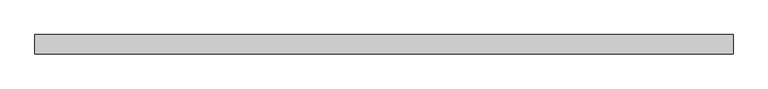
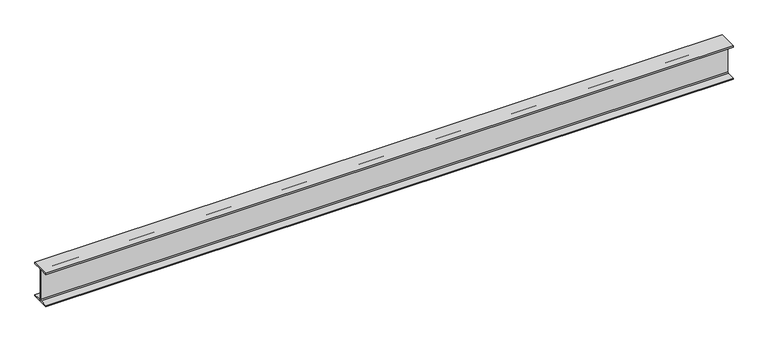
"""IFC4 building model written with IfcOpenShell, lengths in millimetres: beam geometry, Old_Steel Beam_H-KSD3502 : H_SB_ASB_H-350×175x7x11."""

from ifc_helpers import new_model, si_unit, point, frame, frame_2d, origin, place, context, project, spatial, polyline, circle_curve, trimmed, segment, composite_curve, outline, extrude, source, transform, mapped, element, save


def beam_b49fd8c1(model_context):
    return source(origin(), model_context, "Body", "SweptSolid", [
        extrude(outline(composite_curve([segment(polyline([(82.5, -141.5), (82.5, -151.7), (-82.5, -151.7), (-82.5, -141.5), (-11.9, -141.5)]), True, "CONTINUOUS"), segment(trimmed(circle_curve(frame_2d((-11.9, -132.6)), 8.9), [point((-11.9, -141.5))], [point((-3.0, -132.6))], True, "CARTESIAN"), True, "CONTINUOUS"), segment(polyline([(-3.0, -132.6), (-3.0, 132.6)]), True, "CONTINUOUS"), segment(trimmed(circle_curve(frame_2d((-11.9, 132.6)), 8.9), [point((-3.0, 132.6))], [point((-11.9, 141.5))], True, "CARTESIAN"), True, "CONTINUOUS"), segment(polyline([(-11.9, 141.5), (-82.5, 141.5), (-82.5, 151.7), (82.5, 151.7), (82.5, 141.5), (11.9, 141.5)]), True, "CONTINUOUS"), segment(trimmed(circle_curve(frame_2d((11.9, 132.6)), 8.9), [point((11.9, 141.5))], [point((3.0, 132.6))], True, "CARTESIAN"), True, "CONTINUOUS"), segment(polyline([(3.0, 132.6), (3.0, -132.6)]), True, "CONTINUOUS"), segment(trimmed(circle_curve(frame_2d((11.9, -132.6)), 8.9), [point((3.0, -132.6))], [point((11.9, -141.5))], True, "CARTESIAN"), True, "CONTINUOUS"), segment(polyline([(11.9, -141.5), (82.5, -141.5)]), True, "CONTINUOUS")], self_intersect=False)), frame((-2898.0326644, 0.0, 0.0), z_axis=(1.0, 0.0, 0.0), x_axis=(0.0, 1.0, 0.0)), (0.0, 0.0, 1.0), 5920.9678677),
    ])


if __name__ == "__main__":
    model = new_model("IFC4")
    model_context = context("Model", 3, world=origin())
    ifc_project = project(units=[si_unit("LENGTHUNIT", "METRE", prefix="MILLI")], contexts=[model_context])
    site = spatial("IfcSite", under=ifc_project)
    building = spatial("IfcBuilding", under=site)
    placement = place(None, origin())
    beam_shape = beam_b49fd8c1(model_context)
    element("IfcBeam", 1, ObjectType="Old_Steel Beam_H-KSD3502 : H_SB_ASB_H-350×175x7x11", at=placement, inside=building, context=model_context, shape_type="MappedRepresentation", body=[
        mapped(beam_shape, transform((0.0, 0.0, 0.0), x_axis=(1.0, 0.0, 0.0), y_axis=(0.0, 1.0, 0.0), z_axis=(0.0, 0.0, 1.0))),
    ])
    save(model, "model.ifc")

# Revit data of these elements
# Type "Old_Steel Beam_H-KSD3502 : H_SB_ASB_H-350×175x7x11"
#   Width = 17.5 cm
#   Web Thickness = 0.7 cm
#   Web Fillet = 1.4 cm
#   Warping Constant = 282290.0 cm⁶
#   Torsional Moment of Inertia = 19.4042 cm⁴
#   Torsional Modulus = 1.0 cm³
#   Section Area = 63.14 cm²
#   Plastic Modulus weak axis = 174.0 cm³
#   Plastic Modulus strong axis = 868.0 cm³
#   Perimeter = 1.36 m²/m
#   Nominal Weight = 49.60 kgf/m
#   Moment of Inertia weak axis = 984.00 cm⁴
#   Moment of Inertia strong axis = 13600.00 cm⁴
#   Height = 35.0 cm
#   Flange Thickness = 1.1 cm
#   Elastic Modulus weak axis = 112.0 cm³
#   Elastic Modulus strong axis = 775.0 cm³
#   Centroid Vertical = 17.5 cm
#   Centroid Horizontal = 8.75 cm
#   Length [instance default] = 1.5240 m
#   Structural Material [instance default] = Steel, 45-345
#   Assembly Code = ""
# Element 1 (IfcBeam, "Old_Steel Beam_H-KSD3502 : H_SB_ASB_H-350×175x7x11")
#   Structural Material = none
# Materials
#   "Steel, 45-345": class "Metal", colour RGB 189 187 185, transparency 0, Description = "Steel 345 MPa", Cost = 0
